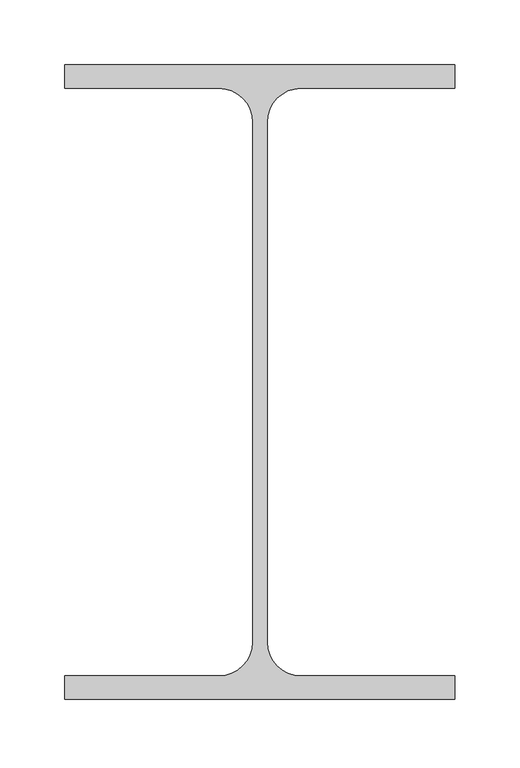
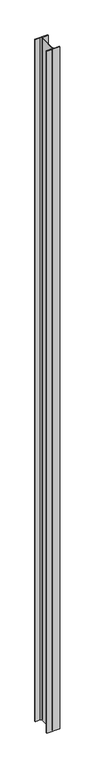
"""IFC4 building model written with IfcOpenShell, lengths in millimetres: column geometry, 0912_Steel Column_H_KSD3502 : H_SC_ASC_H-488x300x11x18."""

from ifc_helpers import new_model, si_unit, point, frame, frame_2d, origin, place, context, project, spatial, polyline, circle_curve, trimmed, segment, composite_curve, outline, extrude, source, transform, mapped, element, save


def column_3ee6d03e(model_context):
    return source(origin(), model_context, "Body", "SweptSolid", [
        extrude(outline(composite_curve([segment(polyline([(150.0, 244.0), (150.0, 226.0), (31.5, 226.0)]), True, "CONTINUOUS"), segment(trimmed(circle_curve(frame_2d((31.5, 200.0)), 26.0), [point((31.5, 226.0))], [point((5.5, 200.0))], True, "CARTESIAN"), True, "CONTINUOUS"), segment(polyline([(5.5, 200.0), (5.5, -200.0)]), True, "CONTINUOUS"), segment(trimmed(circle_curve(frame_2d((31.5, -200.0)), 26.0), [point((5.5, -200.0))], [point((31.5, -226.0))], True, "CARTESIAN"), True, "CONTINUOUS"), segment(polyline([(31.5, -226.0), (150.0, -226.0), (150.0, -244.0), (-150.0, -244.0), (-150.0, -226.0), (-31.5, -226.0)]), True, "CONTINUOUS"), segment(trimmed(circle_curve(frame_2d((-31.5, -200.0)), 26.0), [point((-31.5, -226.0))], [point((-5.5, -200.0))], True, "CARTESIAN"), True, "CONTINUOUS"), segment(polyline([(-5.5, -200.0), (-5.5, 200.0)]), True, "CONTINUOUS"), segment(trimmed(circle_curve(frame_2d((-31.5, 200.0)), 26.0), [point((-5.5, 200.0))], [point((-31.5, 226.0))], True, "CARTESIAN"), True, "CONTINUOUS"), segment(polyline([(-31.5, 226.0), (-150.0, 226.0), (-150.0, 244.0), (150.0, 244.0)]), True, "CONTINUOUS")], self_intersect=False)), frame((0.0, 0.0, 685.9720055), z_axis=(0.0, 0.0, 1.0), x_axis=(1.0, 0.0, 0.0)), (0.0, 0.0, 1.0), 16914.0),
    ])


if __name__ == "__main__":
    model = new_model("IFC4")
    model_context = context("Model", 3, world=origin())
    ifc_project = project(units=[si_unit("LENGTHUNIT", "METRE", prefix="MILLI")], contexts=[model_context])
    site = spatial("IfcSite", under=ifc_project)
    building = spatial("IfcBuilding", under=site)
    placement = place(None, origin())
    column_shape = column_3ee6d03e(model_context)
    element("IfcColumn", 1, ObjectType="0912_Steel Column_H_KSD3502 : H_SC_ASC_H-488x300x11x18", at=placement, inside=building, context=model_context, shape_type="MappedRepresentation", body=[
        mapped(column_shape, transform((0.0, 0.0, 0.0), x_axis=(1.0, 0.0, 0.0), y_axis=(0.0, 1.0, 0.0), z_axis=(0.0, 0.0, 1.0))),
    ])
    save(model, "model.ifc")

# Revit data of these elements
# Type "0912_Steel Column_H_KSD3502 : H_SC_ASC_H-488x300x11x18"
#   H_WM Code_1 = "S01AA002-00001 | Main Steel Structure Fabrication Work | Shelter/Building | Medium Steel - Standard (90KG/M>Weight≥30KG/M) | Material: (   )"
#   H_WM Code_2 = "S03AA028-00001 | Main Steel Structure Erection Work | Shelter/Building | Medium Steel (90KG/M>Weight≥30KG/M) | Material: (   )"
#   H_WM Code_3 = "S01AA010-00001 | Main Steel Structure Fabrication Work | Shelter/Building | Steel Painting/Coating | for Non-Fireproofed Steel Surface, Surface Preparation, Primer, Second & Final Coat | Material: (   )"
#   H_Q'ty Cal Type Tag = "SC-Q2"
#   Width = 30.0 cm
#   Web Thickness = 1.1 cm
#   Web Fillet = 2.6 cm
#   Warping Constant = 4473230.0 cm⁶
#   Torsional Moment of Inertia = 137.492 cm⁴
#   Section Area = 163.5 cm²
#   Plastic Modulus weak axis = 830.0 cm³
#   Plastic Modulus strong axis = 3230.0 cm³
#   Perimeter = 2.11 m²/m
#   Nominal Weight = 128.00 kgf/m
#   Moment of Inertia weak axis = 8110.00 cm⁴
#   Moment of Inertia strong axis = 71000.00 cm⁴
#   Height = 48.8 cm
#   Flange Thickness = 1.8 cm
#   Elastic Modulus weak axis = 541.0 cm³
#   Elastic Modulus strong axis = 2910.0 cm³
#   Centroid Vertical = 24.4 cm
#   Centroid Horizontal = 15.0 cm
#   Structural Material [instance default] = Steel, 45-345
#   Section Name Key = ""
#   Bolt Spacing = 0
#   Assembly Code = ""
# Element 1 (IfcColumn, "0912_Steel Column_H_KSD3502 : H_SC_ASC_H-488x300x11x18")
#   Structural Material = A03AD029-00005_Anchor Bolt (Installation only)_M24
#   Materials on its faces: "A03AD029-00005_Anchor Bolt (Installation only)_M24"
# Materials
#   "Steel, 45-345": class "Metal", colour RGB 189 187 185, transparency 0, Description = "Steel 345 MPa", Cost = 0
#   "A03AD029-00005_Anchor Bolt (Installation only)_M24": class "Unassigned", colour RGB 84 83 81, transparency 0, Cost = 0
